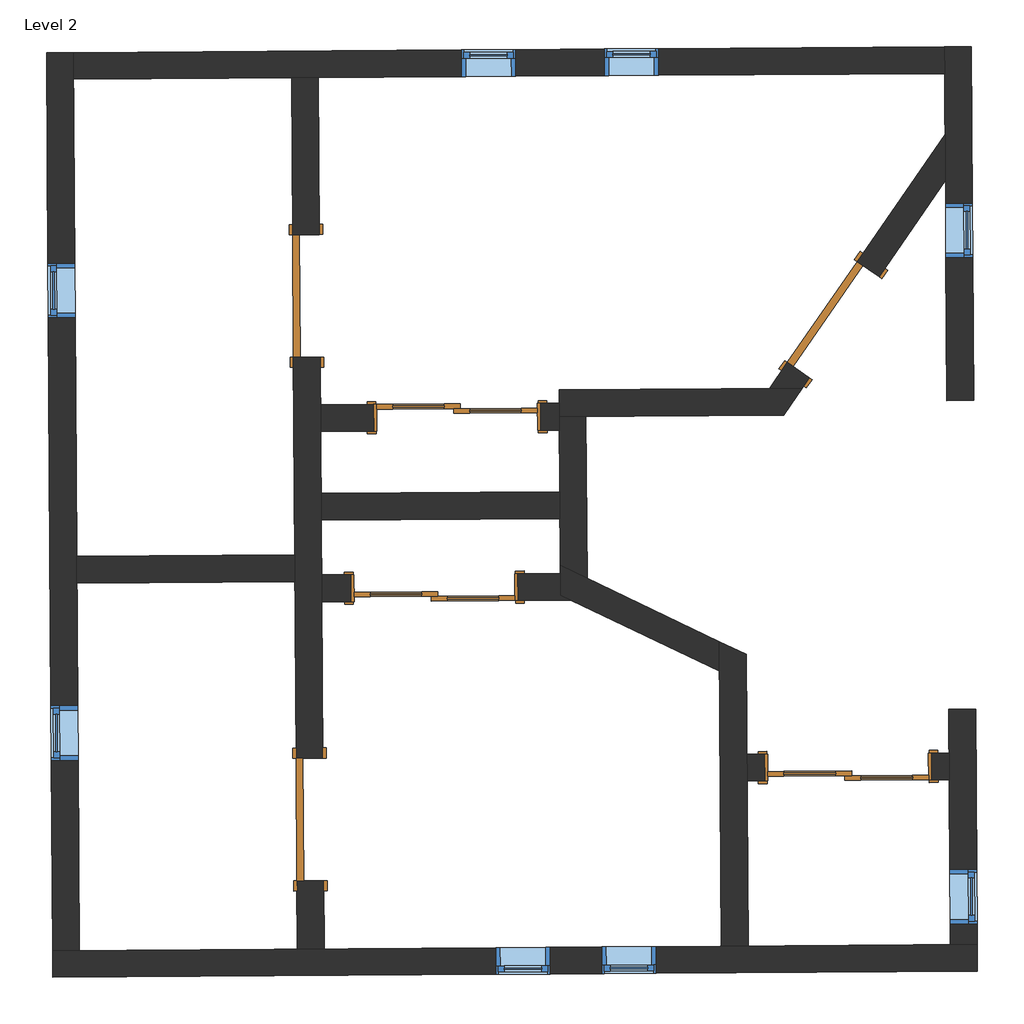
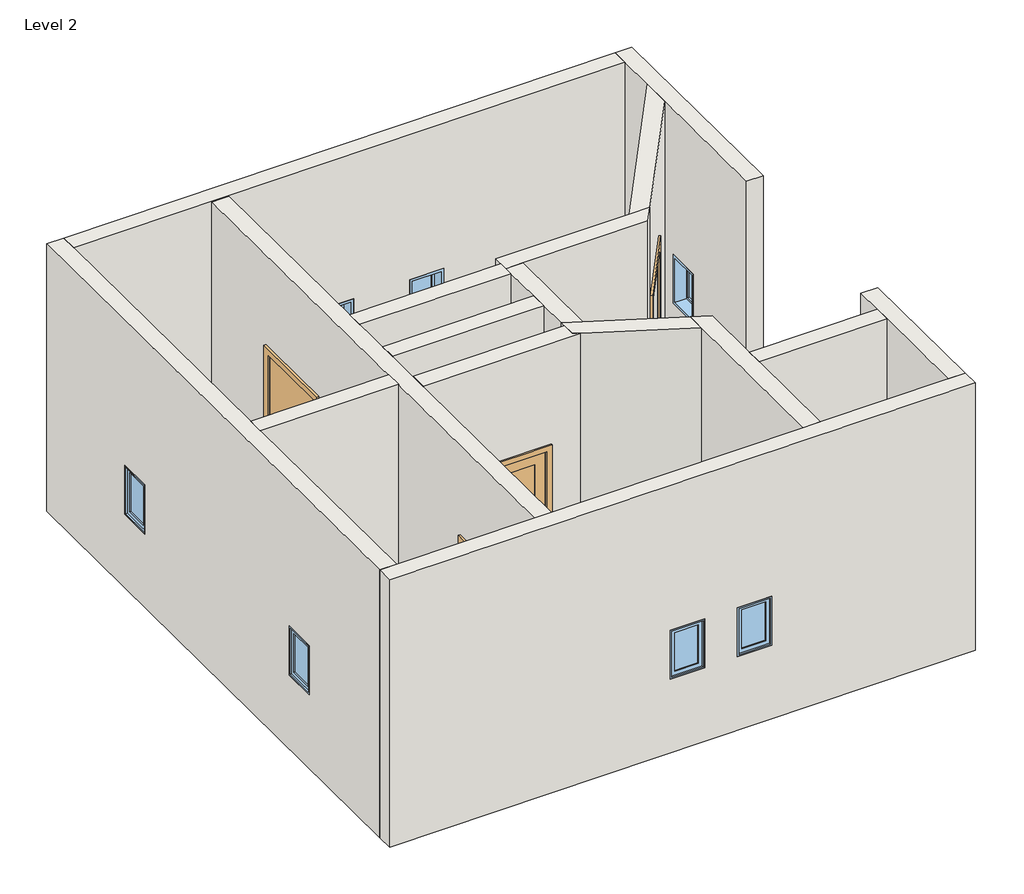
# One storey: 16 walls, 8 windows, 6 doors.
"""IFC4 building model written with IfcOpenShell, lengths in millimetres."""

import ifcopenshell
import ifcopenshell.guid

model = None  # the IFC model being written
_history = None  # IfcOwnerHistory: only IFC2X3 demands one
_inside = {}  # id of a spatial element -> (the spatial element, [elements in it])
_under = {}  # id of a project, library or spatial element -> (it, [spatial elements below it])
_declared = {}  # id of a project -> (the project, [libraries it declares])
_typed = {}  # id of a type object -> (the type object, [elements of that type])
_made_of = {}  # id of a material, layer set ... -> (it, [elements and type objects made of it])


def new_model(schema):
    """Start an empty IFC model of exactly this schema.

    Asked for "IFC4X3", IfcOpenShell would pick the latest addendum, in which some entities
    have other attributes; the version numbers below select the first issue.
    IFC2X3 requires an IfcOwnerHistory on every rooted entity: one is made here for all.
    """
    global model, _history
    if schema == "IFC4X3":
        model = ifcopenshell.file(schema_version=(4, 3, 0, 0))
    else:
        model = ifcopenshell.file(schema=schema)
    _inside.clear()
    _under.clear()
    _declared.clear()
    _typed.clear()
    _made_of.clear()
    _history = None
    if model.schema == "IFC2X3":
        org = make("IfcOrganization", Name="unknown")
        user = make(
            "IfcPersonAndOrganization",
            ThePerson=make("IfcPerson", FamilyName="unknown"),
            TheOrganization=org,
        )
        app = make(
            "IfcApplication",
            ApplicationDeveloper=org,
            Version="unknown",
            ApplicationFullName="unknown",
            ApplicationIdentifier="unknown",
        )
        _history = make(
            "IfcOwnerHistory",
            OwningUser=user,
            OwningApplication=app,
            ChangeAction="ADDED",
            CreationDate=0,
        )
    return model


def make(cls, **values):
    """One entity of the class cls with the attributes given. An attribute that is None is left unset."""
    return model.create_entity(
        cls, **{name: value for name, value in values.items() if value is not None}
    )


def rooted(cls, **values):
    """An entity with a GlobalId (a new one), such as an element, a storey or a relation."""
    return make(cls, GlobalId=ifcopenshell.guid.new(), OwnerHistory=_history, **values)


def si_unit(unit_type, name, prefix=None):
    """IfcSIUnit, for example si_unit("LENGTHUNIT", "METRE", prefix="MILLI")."""
    return make("IfcSIUnit", UnitType=unit_type, Prefix=prefix, Name=name)


def assignment(units):
    """IfcUnitAssignment: the units of a project."""
    return None if units is None else make("IfcUnitAssignment", Units=units)


def point(xyz):
    """IfcCartesianPoint."""
    return None if xyz is None else make("IfcCartesianPoint", Coordinates=xyz)


def direction(xyz):
    """IfcDirection."""
    return None if xyz is None else make("IfcDirection", DirectionRatios=xyz)


def frame(location, z_axis=None, x_axis=None):
    """IfcAxis2Placement3D, a coordinate frame: its origin and axes. An axis left out is left unset."""
    return make(
        "IfcAxis2Placement3D",
        Location=point(location),
        Axis=direction(z_axis),
        RefDirection=direction(x_axis),
    )


def origin():
    """The frame at (0, 0, 0) with its axes left unset."""
    return frame((0.0, 0.0, 0.0))


def origin_with_axes():
    """The frame at (0, 0, 0) with the z axis (0, 0, 1) and the x axis (1, 0, 0) written out."""
    return frame((0.0, 0.0, 0.0), z_axis=(0.0, 0.0, 1.0), x_axis=(1.0, 0.0, 0.0))


def place(relative_to, where):
    """IfcLocalPlacement: puts the frame where relative to a parent placement (None: the world)."""
    return make(
        "IfcLocalPlacement", PlacementRelTo=relative_to, RelativePlacement=where
    )


def context(
    kind, dimensions, precision=None, world=None, true_north=None, identifier=None
):
    """IfcGeometricRepresentationContext, for example the 3D "Model" context."""
    return make(
        "IfcGeometricRepresentationContext",
        ContextIdentifier=identifier,
        ContextType=kind,
        CoordinateSpaceDimension=dimensions,
        Precision=precision,
        WorldCoordinateSystem=world,
        TrueNorth=true_north,
    )


def project(units=None, contexts=None):
    """IfcProject with its units and contexts."""
    return rooted(
        "IfcProject",
        Name="project",
        RepresentationContexts=contexts,
        UnitsInContext=assignment(units),
    )


def spatial(cls, under=None, at=None, **own):
    """A site, building, storey or space (cls), placed at a placement, below another one or the project."""
    s = rooted(cls, ObjectPlacement=at, **own)
    if under is not None:
        _under.setdefault(under.id(), (under, []))[1].append(s)
    return s


def polyline(points):
    """IfcPolyline through the points."""
    return make("IfcPolyline", Points=[point(p) for p in points])


def outline(outer, holes=None, kind="AREA"):
    """IfcArbitraryClosedProfileDef: a profile drawn as a closed curve; with holes, ...WithVoids."""
    if holes is None:
        return make("IfcArbitraryClosedProfileDef", ProfileType=kind, OuterCurve=outer)
    return make(
        "IfcArbitraryProfileDefWithVoids",
        ProfileType=kind,
        OuterCurve=outer,
        InnerCurves=holes,
    )


def extrude(swept, where, along, depth):
    """IfcExtrudedAreaSolid: the profile swept, set in the frame where, extruded along a direction by depth."""
    return make(
        "IfcExtrudedAreaSolid",
        SweptArea=swept,
        Position=where,
        ExtrudedDirection=direction(along),
        Depth=depth,
    )


def faces_of(points, faces, orient=None, outer=None):
    """IfcFace entities. A face is a list of loops; a loop is a list of indices into points, from 0.

    orient and outer hold one flag for each loop. By default every Orientation is true, the
    first loop of a face is its IfcFaceOuterBound and the others are IfcFaceBound.
    """
    made = []
    for i, loops in enumerate(faces):
        bounds = []
        for j, loop in enumerate(loops):
            is_outer = j == 0 if outer is None else outer[i][j]
            bounds.append(
                make(
                    "IfcFaceOuterBound" if is_outer else "IfcFaceBound",
                    Bound=make("IfcPolyLoop", Polygon=[points[k] for k in loop]),
                    Orientation=True if orient is None else orient[i][j],
                )
            )
        made.append(make("IfcFace", Bounds=bounds))
    return made


def faceted_brep(points, faces, orient=None, outer=None, voids=None):
    """IfcFacetedBrep: a solid bounded by flat faces; with voids (closed shells), ...WithVoids."""
    shared = [point(p) for p in points]
    hull = make("IfcClosedShell", CfsFaces=faces_of(shared, faces, orient, outer))
    if voids is None:
        return make("IfcFacetedBrep", Outer=hull)
    return make(
        "IfcFacetedBrepWithVoids",
        Outer=hull,
        Voids=[
            make(cls, CfsFaces=faces_of(shared, fs, o, b)) for cls, fs, o, b in voids
        ],
    )


def shape(context_of_items, identifier, shape_type, items):
    """IfcShapeRepresentation: the items that make up one representation, for example the "Body"."""
    return make(
        "IfcShapeRepresentation",
        ContextOfItems=context_of_items,
        RepresentationIdentifier=identifier,
        RepresentationType=shape_type,
        Items=items,
    )


def source(mapping_origin, context_of_items, identifier, shape_type, items):
    """IfcRepresentationMap: a shape defined once, which mapped items show again and again."""
    return make(
        "IfcRepresentationMap",
        MappingOrigin=mapping_origin,
        MappedRepresentation=shape(context_of_items, identifier, shape_type, items),
    )


def transform(
    local_origin,
    x_axis=None,
    y_axis=None,
    z_axis=None,
    scale=None,
    scale2=None,
    scale3=None,
    uniform=True,
):
    """IfcCartesianTransformationOperator3D, or its non-uniform kind. x_axis, y_axis, z_axis: its Axis1, 2, 3."""
    if uniform:
        return make(
            "IfcCartesianTransformationOperator3D",
            Axis1=direction(x_axis),
            Axis2=direction(y_axis),
            LocalOrigin=point(local_origin),
            Scale=scale,
            Axis3=direction(z_axis),
        )
    return make(
        "IfcCartesianTransformationOperator3DnonUniform",
        Axis1=direction(x_axis),
        Axis2=direction(y_axis),
        LocalOrigin=point(local_origin),
        Scale=scale,
        Axis3=direction(z_axis),
        Scale2=scale2,
        Scale3=scale3,
    )


def mapped(mapping_source, mapping_target):
    """IfcMappedItem: shows the shape of a source again, moved by a transform."""
    return make(
        "IfcMappedItem", MappingSource=mapping_source, MappingTarget=mapping_target
    )


def made_of(thing, what):
    """Note that an element or type object is made of a material, layer set ...; save() writes the relation."""
    if what is not None:
        _made_of.setdefault(what.id(), (what, []))[1].append(thing)
    return thing


def element(
    cls,
    number,
    at=None,
    inside=None,
    cuts=None,
    type_object=None,
    material=None,
    context=None,
    identifier="Body",
    shape_type=None,
    held_by="IfcProductDefinitionShape",
    body=None,
    shapes=None,
    **own,
):
    """One element of the class cls, such as IfcWall. Its Tag is "e" and its number.

    at: its placement. inside: the storey or other place that contains it. cuts: it is an
    opening in that element (IfcRelVoidsElement). A single representation is given by context,
    identifier, shape_type and body (its items); several are given by shapes. held_by: the class
    of the entity that holds the representations. save() writes the other relations.
    """
    e = rooted(cls, Tag="e%d" % number, ObjectPlacement=at, **own)
    if body is not None:
        shapes = [shape(context, identifier, shape_type, body)]
    if shapes is not None:
        e.Representation = make(held_by, Representations=shapes)
    if inside is not None:
        _inside.setdefault(inside.id(), (inside, []))[1].append(e)
    if cuts is not None:
        rooted(
            "IfcRelVoidsElement", RelatingBuildingElement=cuts, RelatedOpeningElement=e
        )
    if type_object is not None:
        _typed.setdefault(type_object.id(), (type_object, []))[1].append(e)
    return made_of(e, material)


def aggregate(whole, parts):
    """IfcRelAggregates: a whole, such as a stair, and the parts it consists of."""
    return rooted("IfcRelAggregates", RelatingObject=whole, RelatedObjects=parts)


def save(model, path):
    """Write the relations noted so far, then the file.

    IfcRelAggregates (storeys below a building ...), IfcRelContainedInSpatialStructure (elements
    in a storey), IfcRelDefinesByType, IfcRelAssociatesMaterial and IfcRelDeclares: one each for
    every whole, place, type object, material and project.
    """
    for whole, parts in _under.values():
        aggregate(whole, parts)
    for where, things in _inside.values():
        rooted(
            "IfcRelContainedInSpatialStructure",
            RelatedElements=things,
            RelatingStructure=where,
        )
    for kind, things in _typed.values():
        rooted("IfcRelDefinesByType", RelatedObjects=things, RelatingType=kind)
    for what, things in _made_of.values():
        rooted("IfcRelAssociatesMaterial", RelatedObjects=things, RelatingMaterial=what)
    for by, libraries in _declared.values():
        rooted("IfcRelDeclares", RelatingContext=by, RelatedDefinitions=libraries)
    model.write(path)


def m_door_interior_double_sliding_2_panel_wood_1200_x_2000mm_2523b4d6(model_context):
    return source(origin(), model_context, "Body", "SweptSolid", [
        extrude(outline(polyline([(480.0, 38.4916667), (94.6, 38.4916667), (94.6, 50.1583333), (480.0, 50.1583333), (480.0, 38.4916667)])), frame((0.0, 0.0, 1014.4), z_axis=(0.0, 0.0, 1.0), x_axis=(1.0, 0.0, 0.0)), (0.0, 0.0, 1.0), 865.6),
        extrude(outline(polyline([(480.0, 38.4916667), (94.6, 38.4916667), (94.6, 50.1583333), (480.0, 50.1583333), (480.0, 38.4916667)])), frame((0.0, 0.0, 230.0), z_axis=(0.0, 0.0, 1.0), x_axis=(1.0, 0.0, 0.0)), (0.0, 0.0, 1.0), 584.4),
        extrude(outline(polyline([(2000.0, -25.4), (0.0, -25.4), (0.0, 600.0), (2000.0, 600.0), (2000.0, -25.4)]), holes=[polyline([(1880.0, 94.6), (1880.0, 480.0), (1014.4, 480.0), (1014.4, 94.6), (1880.0, 94.6)]), polyline([(814.4, 94.6), (814.4, 480.0), (230.0, 480.0), (230.0, 94.6), (814.4, 94.6)])]), frame((0.0, 26.825, 0.0), z_axis=(0.0, 1.0, 0.0), x_axis=(0.0, 0.0, 1.0)), (0.0, 0.0, 1.0), 35.0),
        extrude(outline(polyline([(-94.6, 73.4916667), (-480.0, 73.4916667), (-480.0, 85.1583333), (-94.6, 85.1583333), (-94.6, 73.4916667)])), frame((0.0, 0.0, 1014.4), z_axis=(0.0, 0.0, 1.0), x_axis=(1.0, 0.0, 0.0)), (0.0, 0.0, 1.0), 865.6),
        extrude(outline(polyline([(-94.6, 73.4916667), (-480.0, 73.4916667), (-480.0, 85.1583333), (-94.6, 85.1583333), (-94.6, 73.4916667)])), frame((0.0, 0.0, 230.0), z_axis=(0.0, 0.0, 1.0), x_axis=(1.0, 0.0, 0.0)), (0.0, 0.0, 1.0), 584.4),
        extrude(outline(polyline([(2000.0, -600.0), (0.0, -600.0), (0.0, 25.4), (2000.0, 25.4), (2000.0, -600.0)]), holes=[polyline([(1880.0, -480.0), (1880.0, -94.6), (1014.4, -94.6), (1014.4, -480.0), (1880.0, -480.0)]), polyline([(814.4, -480.0), (814.4, -94.6), (230.0, -94.6), (230.0, -480.0), (814.4, -480.0)])]), frame((0.0, 61.825, 0.0), z_axis=(0.0, 1.0, 0.0), x_axis=(0.0, 0.0, 1.0)), (0.0, 0.0, 1.0), 35.0),
        extrude(outline(polyline([(0.0, 600.0), (0.0, 625.0), (2025.0, 625.0), (2025.0, -625.0), (0.0, -625.0), (0.0, -600.0), (2000.0, -600.0), (2000.0, 600.0), (0.0, 600.0)])), frame((0.0, -103.175, 0.0), z_axis=(0.0, 1.0, 0.0), x_axis=(0.0, 0.0, 1.0)), (0.0, 0.0, 1.0), 200.0),
        extrude(outline(polyline([(0.0, 606.35), (0.0, 671.35), (2071.35, 671.35), (2071.35, -671.35), (0.0, -671.35), (0.0, -606.35), (2006.35, -606.35), (2006.35, 606.35), (0.0, 606.35)])), frame((0.0, -123.175, 0.0), z_axis=(0.0, 1.0, 0.0), x_axis=(0.0, 0.0, 1.0)), (0.0, 0.0, 1.0), 20.0),
        extrude(outline(polyline([(0.0, 606.35), (0.0, 671.35), (2071.35, 671.35), (2071.35, -671.35), (0.0, -671.35), (0.0, -606.35), (2006.35, -606.35), (2006.35, 606.35), (0.0, 606.35)])), frame((0.0, 96.825, 0.0), z_axis=(0.0, 1.0, 0.0), x_axis=(0.0, 0.0, 1.0)), (0.0, 0.0, 1.0), 20.0),
    ])


def m_single_flush_0915_x_2134mm_6a9e8738(model_context):
    return source(origin(), model_context, "Body", "SweptSolid", [
        extrude(outline(polyline([(2210.0, -533.5), (0.0, -533.5), (0.0, -457.5), (2134.0, -457.5), (2134.0, 457.5), (0.0, 457.5), (0.0, 533.5), (2210.0, 533.5), (2210.0, -533.5)])), frame((0.0, 100.0, 0.0), z_axis=(0.0, 1.0, 0.0), x_axis=(0.0, 0.0, 1.0)), (0.0, 0.0, 1.0), 25.0),
        extrude(outline(polyline([(2210.0, 533.5), (2210.0, -533.5), (0.0, -533.5), (0.0, -457.5), (2134.0, -457.5), (2134.0, 457.5), (0.0, 457.5), (0.0, 533.5), (2210.0, 533.5)])), frame((0.0, -125.0, 0.0), z_axis=(0.0, 1.0, 0.0), x_axis=(0.0, 0.0, 1.0)), (0.0, 0.0, 1.0), 25.0),
        extrude(outline(polyline([(457.5, 49.0), (-457.5, 49.0), (-457.5, 100.0), (457.5, 100.0), (457.5, 49.0)])), origin_with_axes(), (0.0, 0.0, 1.0), 2134.0),
    ])


def m_single_flush_0915_x_2134mm_727434cd(model_context):
    return source(origin(), model_context, "Body", "SweptSolid", [
        extrude(outline(polyline([(2210.0, -533.5), (0.0, -533.5), (0.0, -457.5), (2134.0, -457.5), (2134.0, 457.5), (0.0, 457.5), (0.0, 533.5), (2210.0, 533.5), (2210.0, -533.5)])), frame((0.0, -125.0, 0.0), z_axis=(0.0, 1.0, 0.0), x_axis=(0.0, 0.0, 1.0)), (0.0, 0.0, 1.0), 25.0),
        extrude(outline(polyline([(2210.0, 533.5), (2210.0, -533.5), (0.0, -533.5), (0.0, -457.5), (2134.0, -457.5), (2134.0, 457.5), (0.0, 457.5), (0.0, 533.5), (2210.0, 533.5)])), frame((0.0, 100.0, 0.0), z_axis=(0.0, 1.0, 0.0), x_axis=(0.0, 0.0, 1.0)), (0.0, 0.0, 1.0), 25.0),
        extrude(outline(polyline([(457.5, -49.0), (457.5, -100.0), (-457.5, -100.0), (-457.5, -49.0), (457.5, -49.0)])), origin_with_axes(), (0.0, 0.0, 1.0), 2134.0),
    ])


def m_fixed_0406_x_0610mm_8205b201(model_context):
    return source(origin(), model_context, "Body", "SweptSolid", [
        extrude(outline(polyline([(-140.0, 78.0), (140.0, 78.0), (140.0, 66.0), (-140.0, 66.0), (-140.0, 78.0)])), frame((0.0, 0.0, 978.0), z_axis=(0.0, 0.0, 1.0), x_axis=(1.0, 0.0, 0.0)), (0.0, 0.0, 1.0), 484.0),
        extrude(outline(polyline([(1506.0, -184.0), (934.0, -184.0), (934.0, 184.0), (1506.0, 184.0), (1506.0, -184.0)]), holes=[polyline([(1462.0, -140.0), (1462.0, 140.0), (978.0, 140.0), (978.0, -140.0), (1462.0, -140.0)])]), frame((0.0, 50.0, 0.0), z_axis=(0.0, 1.0, 0.0), x_axis=(0.0, 0.0, 1.0)), (0.0, 0.0, 1.0), 44.0),
        extrude(outline(polyline([(1525.0, -203.0), (915.0, -203.0), (915.0, 203.0), (1525.0, 203.0), (1525.0, -203.0)]), holes=[polyline([(1506.0, -184.0), (1506.0, 184.0), (934.0, 184.0), (934.0, -184.0), (1506.0, -184.0)])]), frame((0.0, 50.0, 0.0), z_axis=(0.0, 1.0, 0.0), x_axis=(0.0, 0.0, 1.0)), (0.0, 0.0, 1.0), 63.0),
        extrude(outline(polyline([(1525.0, -203.0), (915.0, -203.0), (915.0, 203.0), (1525.0, 203.0), (1525.0, -203.0)]), holes=[polyline([(1493.0, -171.0), (1493.0, 171.0), (947.0, 171.0), (947.0, -171.0), (1493.0, -171.0)])]), frame((0.0, -87.0, 0.0), z_axis=(0.0, 1.0, 0.0), x_axis=(0.0, 0.0, 1.0)), (0.0, 0.0, 1.0), 137.0),
    ])


model = new_model("IFC4")

# Units and contexts
model_context = context("Model", 3, world=origin())
ifc_project = project(units=[si_unit("LENGTHUNIT", "METRE", prefix="MILLI")], contexts=[model_context])

# Site, building, storey
site = spatial("IfcSite", under=ifc_project)
building = spatial("IfcBuilding", under=site)
storey = spatial("IfcBuildingStorey", under=building, Name="Level 2", Elevation=3048.0)

# Doors
placement = place(None, origin())
m_door_interior_double_sliding_2_panel_wood_1200_x_2000mm_shape = m_door_interior_double_sliding_2_panel_wood_1200_x_2000mm_2523b4d6(model_context)
element("IfcDoor", 1, ObjectType="M_Door-Interior-Double-Sliding-2_Panel-Wood : 1200 x 2000mm", at=placement, inside=storey, context=model_context, shape_type="MappedRepresentation", body=[
    mapped(m_door_interior_double_sliding_2_panel_wood_1200_x_2000mm_shape, transform((-71680.7342744, -7306.8218345, 3048.0), x_axis=(0.9999777944135733, 0.006664133834601911, 0.0), y_axis=(-0.006664133834601911, 0.9999777944135733, 0.0), z_axis=(0.0, 0.0, 1.0))),
])
element("IfcDoor", 2, ObjectType="M_Door-Interior-Double-Sliding-2_Panel-Wood : 1200 x 2000mm", at=placement, inside=storey, context=model_context, shape_type="MappedRepresentation", body=[
    mapped(m_door_interior_double_sliding_2_panel_wood_1200_x_2000mm_shape, transform((-71850.8195491, -8585.0827996, 3048.0), x_axis=(-0.9999777944135733, -0.006664133834601911, 0.0), y_axis=(0.006664133834601911, -0.9999777944135733, 0.0), z_axis=(0.0, 0.0, 1.0))),
])
element("IfcDoor", 3, ObjectType="M_Door-Interior-Double-Sliding-2_Panel-Wood : 1200 x 2000mm", at=placement, inside=storey, context=model_context, shape_type="MappedRepresentation", body=[
    mapped(m_door_interior_double_sliding_2_panel_wood_1200_x_2000mm_shape, transform((-68760.728221, -9924.4626813, 3048.0), x_axis=(-0.9999777944135733, -0.006664133834601911, 0.0), y_axis=(0.006664133834601911, -0.9999777944135733, 0.0), z_axis=(0.0, 0.0, 1.0))),
])
m_single_flush_0915_x_2134mm_shape = m_single_flush_0915_x_2134mm_6a9e8738(model_context)
element("IfcDoor", 4, ObjectType="M_Single-Flush : 0915 x 2134mm", at=placement, inside=storey, context=model_context, shape_type="MappedRepresentation", body=[
    mapped(m_single_flush_0915_x_2134mm_shape, transform((-68872.1991372, -6581.0027274, 3048.0), x_axis=(0.5681047608958888, 0.8229562446736918, 0.0), y_axis=(-0.8229562446736918, 0.5681047608958888, 0.0), z_axis=(0.0, 0.0, 1.0))),
])
element("IfcDoor", 5, ObjectType="M_Single-Flush : 0915 x 2134mm", at=placement, inside=storey, context=model_context, shape_type="MappedRepresentation", body=[
    mapped(m_single_flush_0915_x_2134mm_shape, transform((-72805.9812977, -6403.1730367, 3048.0), x_axis=(-0.0066641338345986775, 0.9999777944135734, 0.0), y_axis=(-0.9999777944135734, -0.0066641338345986775, 0.0), z_axis=(0.0, 0.0, 1.0))),
])
m_single_flush_0915_x_2134mm_2_shape = m_single_flush_0915_x_2134mm_727434cd(model_context)
element("IfcDoor", 6, ObjectType="M_Single-Flush : 0915 x 2134mm", at=placement, inside=storey, context=model_context, shape_type="MappedRepresentation", body=[
    mapped(m_single_flush_0915_x_2134mm_2_shape, transform((-72779.9238848, -10313.1836822, 3048.0), x_axis=(0.0066641338345986775, -0.9999777944135734, 0.0), y_axis=(0.9999777944135734, 0.0066641338345986775, 0.0), z_axis=(0.0, 0.0, 1.0))),
])

# Walls
element("IfcWall", 7, ObjectType="Generic - 200mm", at=placement, inside=storey, context=model_context, shape_type="Brep", body=[
    faceted_brep([(-67796.791513, -11246.7961526, 3048.0), (-67996.7870719, -11248.1289794, 3048.0), (-69506.9597289, -11258.1931955, 3048.0), (-69706.9552878, -11259.5260223, 3048.0), (-72673.4832208, -11279.2958005, 3048.0), (-72873.4787797, -11280.6286272, 3048.0), (-74502.2426112, -11291.4831684, 3048.0), (-74702.2381701, -11292.8159952, 3048.0), (-74702.2381701, -11292.8159952, 6372.225), (-74502.2426112, -11291.4831684, 6372.225), (-69706.9552878, -11259.5260223, 6372.225), (-69506.9597289, -11258.1931955, 6372.225), (-67996.7870719, -11248.1289794, 6372.225), (-67796.791513, -11246.7961526, 6372.225), (-70987.223762, -11268.0580922, 3963.0), (-70987.223762, -11268.0580922, 4573.0), (-71393.2147465, -11270.7637306, 4573.0), (-71393.2147465, -11270.7637306, 3963.0), (-70195.592889, -11262.782441, 3963.0), (-70195.592889, -11262.782441, 4573.0), (-70601.5838736, -11265.4880793, 4573.0), (-70601.5838736, -11265.4880793, 3963.0), (-67795.4586862, -11446.7917115, 3048.0), (-67795.4586862, -11446.7917115, 6372.225), (-74700.9053433, -11492.8115541, 6372.225), (-74700.9053433, -11492.8115541, 3048.0), (-70985.8909352, -11468.0536511, 3963.0), (-71391.8819198, -11470.7592894, 3963.0), (-71391.8819198, -11470.7592894, 4573.0), (-70985.8909352, -11468.0536511, 4573.0), (-70194.2600623, -11462.7779999, 3963.0), (-70600.2510468, -11465.4836382, 3963.0), (-70600.2510468, -11465.4836382, 4573.0), (-70194.2600623, -11462.7779999, 4573.0)], [[[0, 1, 2, 3, 4, 5, 6, 7, 8, 9, 10, 11, 12, 13], [14, 15, 16, 17], [18, 19, 20, 21]], [[22, 23, 24, 25], [26, 27, 28, 29], [30, 31, 32, 33]], [[8, 7, 25, 24]], [[0, 13, 23, 22]], [[15, 14, 26, 29]], [[16, 15, 29, 28]], [[17, 16, 28, 27]], [[14, 17, 27, 26]], [[19, 18, 30, 33]], [[20, 19, 33, 32]], [[21, 20, 32, 31]], [[18, 21, 31, 30]], [[7, 6, 5, 4, 3, 2, 1, 0, 22, 25]], [[13, 12, 11, 10, 9, 8, 24, 23]]]),
])
element("IfcWall", 8, ObjectType="Generic - 200mm", at=placement, inside=storey, context=model_context, shape_type="Brep", body=[
    faceted_brep([(-74502.2426112, -11291.4831684, 3048.0), (-74520.5249623, -8548.1491441, 3048.0), (-74521.857789, -8348.1535853, 3048.0), (-74545.5968003, -4786.0276291, 3048.0), (-74546.9296271, -4586.0320702, 3048.0), (-74546.9296271, -4586.0320702, 6372.225), (-74545.5968003, -4786.0276291, 6372.225), (-74521.857789, -8348.1535853, 6372.225), (-74520.5249623, -8548.1491441, 6372.225), (-74502.2426112, -11291.4831684, 6372.225), (-74533.7386405, -6565.3881165, 3963.0), (-74533.7386405, -6565.3881165, 4573.0), (-74536.4442789, -6159.3971319, 4573.0), (-74536.4442789, -6159.3971319, 3963.0), (-74511.7136445, -9870.3197839, 3963.0), (-74511.7136445, -9870.3197839, 4573.0), (-74514.4192829, -9464.3287994, 4573.0), (-74514.4192829, -9464.3287994, 3963.0), (-74702.2381701, -11292.8159952, 3048.0), (-74702.2381701, -11292.8159952, 6372.225), (-74746.9251859, -4587.364897, 6372.225), (-74746.9251859, -4587.364897, 3048.0), (-74733.7341994, -6566.7209432, 3963.0), (-74736.4398378, -6160.7299587, 3963.0), (-74736.4398378, -6160.7299587, 4573.0), (-74733.7341994, -6566.7209432, 4573.0), (-74711.7092034, -9871.6526107, 3963.0), (-74714.4148417, -9465.6616262, 3963.0), (-74714.4148417, -9465.6616262, 4573.0), (-74711.7092034, -9871.6526107, 4573.0)], [[[0, 1, 2, 3, 4, 5, 6, 7, 8, 9], [10, 11, 12, 13], [14, 15, 16, 17]], [[18, 19, 20, 21], [22, 23, 24, 25], [26, 27, 28, 29]], [[4, 3, 2, 1, 0, 18, 21]], [[9, 8, 7, 6, 5, 20, 19]], [[0, 9, 19, 18]], [[5, 4, 21, 20]], [[11, 10, 22, 25]], [[12, 11, 25, 24]], [[13, 12, 24, 23]], [[10, 13, 23, 22]], [[15, 14, 26, 29]], [[16, 15, 29, 28]], [[17, 16, 28, 27]], [[14, 17, 27, 26]]]),
])
element("IfcWall", 9, ObjectType="Generic - 200mm", at=placement, inside=storey, context=model_context, shape_type="Brep", body=[
    faceted_brep([(-74545.5968003, -4786.0276291, 3048.0), (-72916.8329687, -4775.1730879, 3048.0), (-72716.8374099, -4773.8402611, 3048.0), (-68040.141261, -4742.67344, 3048.0), (-68040.141261, -4742.67344, 6372.225), (-74545.5968003, -4786.0276291, 6372.225), (-70581.4848277, -4759.6096698, 3963.0), (-70581.4848277, -4759.6096698, 4573.0), (-70175.4938431, -4756.9040314, 4573.0), (-70175.4938431, -4756.9040314, 3963.0), (-71648.2611388, -4766.7189677, 3963.0), (-71648.2611388, -4766.7189677, 4573.0), (-71242.2701542, -4764.0133294, 4573.0), (-71242.2701542, -4764.0133294, 3963.0), (-74546.9296271, -4586.0320702, 3048.0), (-74546.9296271, -4586.0320702, 6372.225), (-68041.4740877, -4542.6778811, 6372.225), (-68041.4740877, -4542.6778811, 3048.0), (-70582.8176544, -4559.6141109, 3963.0), (-70176.8266699, -4556.9084725, 3963.0), (-70176.8266699, -4556.9084725, 4573.0), (-70582.8176544, -4559.6141109, 4573.0), (-71649.5939655, -4566.7234088, 3963.0), (-71243.602981, -4564.0177705, 3963.0), (-71243.602981, -4564.0177705, 4573.0), (-71649.5939655, -4566.7234088, 4573.0)], [[[0, 1, 2, 3, 4, 5], [6, 7, 8, 9], [10, 11, 12, 13]], [[14, 15, 16, 17], [18, 19, 20, 21], [22, 23, 24, 25]], [[3, 2, 1, 0, 14, 17]], [[5, 4, 16, 15]], [[0, 5, 15, 14]], [[7, 6, 18, 21]], [[8, 7, 21, 20]], [[9, 8, 20, 19]], [[6, 9, 19, 18]], [[11, 10, 22, 25]], [[12, 11, 25, 24]], [[13, 12, 24, 23]], [[10, 13, 23, 22]], [[4, 3, 17, 16]]]),
])
element("IfcWall", 10, ObjectType="Generic - 200mm", at=placement, inside=storey, context=model_context, shape_type="Brep", body=[
    faceted_brep([(-68041.4740877, -4542.6778811, 3048.0), (-68040.141261, -4742.67344, 3048.0), (-68037.1248916, -5195.2907613, 3048.0), (-68034.801179, -5543.9723775, 3048.0), (-68023.8607483, -7185.6242487, 3048.0), (-68023.8607483, -7185.6242487, 6372.225), (-68034.801179, -5543.9723775, 6372.225), (-68037.1248916, -5195.2907613, 6372.225), (-68040.141261, -4742.67344, 6372.225), (-68041.4740877, -4542.6778811, 6372.225), (-68033.6870305, -5711.1544624, 3963.0), (-68033.6870305, -5711.1544624, 4573.0), (-68030.9813921, -6117.1454469, 4573.0), (-68030.9813921, -6117.1454469, 3963.0), (-67841.4785288, -4541.3450544, 3048.0), (-67841.4785288, -4541.3450544, 6372.225), (-67823.8651894, -7184.2914219, 6372.225), (-67823.8651894, -7184.2914219, 3048.0), (-67833.6914716, -5709.8216356, 3963.0), (-67830.9858333, -6115.8126201, 3963.0), (-67830.9858333, -6115.8126201, 4573.0), (-67833.6914716, -5709.8216356, 4573.0)], [[[0, 1, 2, 3, 4, 5, 6, 7, 8, 9], [10, 11, 12, 13]], [[14, 15, 16, 17], [18, 19, 20, 21]], [[4, 3, 2, 1, 0, 14, 17]], [[5, 4, 17, 16]], [[9, 8, 7, 6, 5, 16, 15]], [[11, 10, 18, 21]], [[12, 11, 21, 20]], [[13, 12, 20, 19]], [[10, 13, 19, 18]], [[0, 9, 15, 14]]]),
])
element("IfcWall", 11, ObjectType="Generic - 200mm", at=placement, inside=storey, context=model_context, shape_type="Brep", body=[
    faceted_brep([(-67796.791513, -11246.7961526, 3048.0), (-67808.4990553, -9490.0363627, 3048.0), (-67808.4990553, -9490.0363627, 6372.225), (-67796.791513, -11246.7961526, 6372.225), (-67800.5247608, -10686.6085922, 3963.0), (-67797.8191224, -11092.5995767, 3963.0), (-67797.8191224, -11092.5995767, 4573.0), (-67800.5247608, -10686.6085922, 4573.0), (-67996.7870719, -11248.1289794, 3048.0), (-67996.7870719, -11248.1289794, 6372.225), (-68004.9966377, -10016.2534232, 6372.225), (-68006.3294645, -9816.2578643, 6372.225), (-68008.4946142, -9491.3691895, 6372.225), (-68008.4946142, -9491.3691895, 3048.0), (-68006.3294645, -9816.2578643, 3048.0), (-68004.9966377, -10016.2534232, 3048.0), (-68000.5203197, -10687.9414189, 3963.0), (-68000.5203197, -10687.9414189, 4573.0), (-67997.8146813, -11093.9324035, 4573.0), (-67997.8146813, -11093.9324035, 3963.0)], [[[0, 1, 2, 3], [4, 5, 6, 7]], [[8, 9, 10, 11, 12, 13, 14, 15], [16, 17, 18, 19]], [[1, 0, 8, 15, 14, 13]], [[2, 1, 13, 12]], [[3, 2, 12, 11, 10, 9]], [[0, 3, 9, 8]], [[17, 16, 4, 7]], [[18, 17, 7, 6]], [[19, 18, 6, 5]], [[16, 19, 5, 4]]]),
])
element("IfcWall", 12, ObjectType="Generic - 200mm", at=placement, inside=storey, context=model_context, shape_type="Brep", body=[
    faceted_brep([(-72876.872823, -10771.3399365, 5182.0), (-72876.872823, -10771.3399365, 3048.0), (-72873.4787797, -11280.6286272, 3048.0), (-72873.4787797, -11280.6286272, 6363.9898437), (-72916.8329687, -4775.1730879, 6363.9898437), (-72916.8329687, -4775.1730879, 3048.0), (-72909.0279183, -5946.3496092, 3048.0), (-72909.0279183, -5946.3496092, 5182.0), (-72902.9302359, -6861.3292911, 5182.0), (-72902.9302359, -6861.3292911, 3048.0), (-72893.0939575, -8337.2990441, 3048.0), (-72891.7611307, -8537.294603, 3048.0), (-72882.9705055, -9856.3602547, 3048.0), (-72882.9705055, -9856.3602547, 5182.0), (-72673.4832208, -11279.2958005, 3048.0), (-72676.8772642, -10770.0071098, 3048.0), (-72676.8772642, -10770.0071098, 5182.0), (-72682.9749466, -9855.0274279, 5182.0), (-72682.9749466, -9855.0274279, 3048.0), (-72690.7556283, -8687.5075204, 3048.0), (-72692.0884551, -8487.5119615, 3048.0), (-72694.8124138, -8078.7719286, 3048.0), (-72696.1452406, -7878.7763697, 3048.0), (-72699.2240704, -7416.7866287, 3048.0), (-72700.5568972, -7216.7910698, 3048.0), (-72702.934677, -6859.9964643, 3048.0), (-72702.934677, -6859.9964643, 5182.0), (-72709.0323595, -5945.0167824, 5182.0), (-72709.0323595, -5945.0167824, 3048.0), (-72716.8374099, -4773.8402611, 3048.0), (-72716.8374099, -4773.8402611, 6363.9898437), (-72673.4832208, -11279.2958005, 6363.9898437)], [[[0, 1, 2, 3, 4, 5, 6, 7, 8, 9, 10, 11, 12, 13]], [[14, 15, 16, 17, 18, 19, 20, 21, 22, 23, 24, 25, 26, 27, 28, 29, 30, 31]], [[3, 2, 14, 31]], [[5, 4, 30, 29]], [[7, 6, 28, 27]], [[8, 7, 27, 26]], [[9, 8, 26, 25]], [[16, 15, 1, 0]], [[17, 16, 0, 13]], [[18, 17, 13, 12]], [[29, 28, 6, 5]], [[2, 1, 15, 14]], [[12, 11, 10, 9, 25, 24, 23, 22, 21, 20, 19, 18]], [[4, 3, 31, 30]]]),
])
element("IfcWall", 13, ObjectType="Generic - 200mm", at=placement, inside=storey, context=model_context, shape_type="Brep", body=[
    faceted_brep([(-70918.7300364, -7304.9186941, 3048.0), (-70718.7344775, -7303.5858673, 3048.0), (-69242.7105492, -7293.7492279, 3048.0), (-69242.7105492, -7293.7492279, 6372.225), (-70718.7344775, -7303.5858673, 6372.225), (-70918.7300364, -7304.9186941, 6372.225), (-70920.0628632, -7104.9231352, 3048.0), (-70920.0628632, -7104.9231352, 6372.225), (-69348.1544742, -7094.4474947, 6372.225), (-69104.004978, -7092.8204136, 6372.225), (-69104.004978, -7092.8204136, 3048.0), (-69348.1544742, -7094.4474947, 3048.0), (-70919.3964498, -7204.9209146, 3048.0), (-70919.3964498, -7204.9209146, 6372.225)], [[[0, 1, 2, 3, 4, 5]], [[6, 7, 8, 9, 10, 11]], [[2, 1, 0, 12, 6, 11, 10]], [[5, 4, 3, 9, 8, 7, 13]], [[3, 2, 10, 9]], [[0, 5, 13, 7, 6, 12]]]),
])
element("IfcWall", 14, ObjectType="Generic - 200mm", at=placement, inside=storey, context=model_context, shape_type="Brep", body=[
    faceted_brep([(-68529.9955846, -6261.3107215, 5182.0), (-68529.9955846, -6261.3107215, 3048.0), (-68034.801179, -5543.9723775, 3048.0), (-68034.801179, -5543.9723775, 6372.225), (-69104.004978, -7092.8204136, 6372.225), (-69104.004978, -7092.8204136, 3048.0), (-69049.8114408, -7014.3156854, 3048.0), (-69049.8114408, -7014.3156854, 5182.0), (-68037.1248916, -5195.2907613, 3048.0), (-68694.5868335, -6147.6897693, 3048.0), (-68694.5868335, -6147.6897693, 5182.0), (-69214.4026897, -6900.6947332, 5182.0), (-69214.4026897, -6900.6947332, 3048.0), (-69348.1544742, -7094.4474947, 3048.0), (-69348.1544742, -7094.4474947, 6372.225), (-68037.1248916, -5195.2907613, 6372.225)], [[[0, 1, 2, 3, 4, 5, 6, 7]], [[8, 9, 10, 11, 12, 13, 14, 15]], [[6, 5, 13, 12]], [[2, 1, 9, 8]], [[4, 3, 15, 14]], [[5, 4, 14, 13]], [[3, 2, 8, 15]], [[10, 9, 1, 0]], [[11, 10, 0, 7]], [[12, 11, 7, 6]]]),
])
element("IfcWall", 15, ObjectType="Generic - 200mm", at=placement, inside=storey, context=model_context, shape_type="Brep", body=[
    faceted_brep([(-69722.1165345, -8984.5251792, 3048.0), (-69720.6343726, -9206.9290273, 3048.0), (-69706.9552878, -11259.5260223, 3048.0), (-69706.9552878, -11259.5260223, 6372.225), (-69720.6343726, -9206.9290273, 6372.225), (-69722.1165345, -8984.5251792, 6372.225), (-69521.4726109, -9080.4818591, 3048.0), (-69521.4726109, -9080.4818591, 6372.225), (-69516.5021215, -9826.3220805, 6372.225), (-69515.1692948, -10026.3176394, 6372.225), (-69506.9597289, -11258.1931955, 6372.225), (-69506.9597289, -11258.1931955, 3048.0), (-69515.1692948, -10026.3176394, 3048.0), (-69516.5021215, -9826.3220805, 3048.0)], [[[0, 1, 2, 3, 4, 5]], [[6, 7, 8, 9, 10, 11, 12, 13]], [[2, 1, 0, 6, 13, 12, 11]], [[5, 4, 3, 10, 9, 8, 7]], [[3, 2, 11, 10]], [[0, 5, 7, 6]]]),
])
element("IfcWall", 16, ObjectType="Generic - 200mm", at=placement, inside=storey, context=model_context, shape_type="Brep", body=[
    faceted_brep([(-70909.8446957, -8638.1967565, 3048.0), (-70832.629476, -8675.1244441, 3048.0), (-69720.6343726, -9206.9290273, 3048.0), (-69720.6343726, -9206.9290273, 6372.225), (-70832.629476, -8675.1244441, 6372.225), (-70909.8446957, -8638.1967565, 6372.225), (-70911.3268576, -8415.7929084, 3048.0), (-70911.3268576, -8415.7929084, 6372.225), (-70710.682934, -8511.7495883, 6372.225), (-69722.1165345, -8984.5251792, 6372.225), (-69722.1165345, -8984.5251792, 3048.0), (-70710.682934, -8511.7495883, 3048.0), (-70910.9280077, -8475.6418063, 3048.0), (-70910.9280077, -8475.6418063, 6372.225)], [[[0, 1, 2, 3, 4, 5]], [[6, 7, 8, 9, 10, 11]], [[2, 1, 0, 12, 6, 11, 10]], [[5, 4, 3, 9, 8, 7, 13]], [[3, 2, 10, 9]], [[0, 5, 13, 7, 6, 12]]]),
])
element("IfcWall", 17, ObjectType="Generic - 200mm", at=placement, inside=storey, context=model_context, shape_type="Brep", body=[
    faceted_brep([(-70918.7300364, -7304.9186941, 3048.0), (-70918.063623, -7404.9164735, 3048.0), (-70914.9847932, -7866.9062145, 3048.0), (-70913.6519664, -8066.9017734, 3048.0), (-70911.3268576, -8415.7929084, 3048.0), (-70911.3268576, -8415.7929084, 6372.225), (-70913.6519664, -8066.9017734, 6372.225), (-70914.9847932, -7866.9062145, 6372.225), (-70918.063623, -7404.9164735, 6372.225), (-70918.7300364, -7304.9186941, 6372.225), (-70718.7344775, -7303.5858673, 3048.0), (-70718.7344775, -7303.5858673, 6372.225), (-70710.682934, -8511.7495883, 6372.225), (-70710.682934, -8511.7495883, 3048.0)], [[[0, 1, 2, 3, 4, 5, 6, 7, 8, 9]], [[10, 11, 12, 13]], [[4, 3, 2, 1, 0, 10, 13]], [[9, 8, 7, 6, 5, 12, 11]], [[0, 9, 11, 10]], [[5, 4, 13, 12]]]),
])
element("IfcWall", 18, ObjectType="Generic - 200mm", at=placement, inside=storey, context=model_context, shape_type="SweptSolid", body=[
    extrude(outline(polyline([(-74521.857789, -8348.1535853), (-72893.0939575, -8337.2990441), (-72891.7611307, -8537.294603), (-74520.5249623, -8548.1491441), (-74521.857789, -8348.1535853)])), frame((0.0, 0.0, 3048.0), z_axis=(0.0, 0.0, 1.0), x_axis=(1.0, 0.0, 0.0)), (0.0, 0.0, 1.0), 3324.225),
])
element("IfcWall", 19, ObjectType="Generic - 200mm", at=placement, inside=storey, context=model_context, shape_type="Brep", body=[
    faceted_brep([(-72700.5568972, -7216.7910698, 6372.225), (-70919.3964498, -7204.9209146, 6372.225), (-70919.3964498, -7204.9209146, 3048.0), (-71056.3934076, -7205.833901, 3048.0), (-71056.3934076, -7205.833901, 5073.0), (-72306.3656506, -7214.1640682, 5073.0), (-72306.3656506, -7214.1640682, 3048.0), (-72700.5568972, -7216.7910698, 3048.0), (-70918.063623, -7404.9164735, 6372.225), (-72699.2240704, -7416.7866287, 6372.225), (-72699.2240704, -7416.7866287, 3048.0), (-72305.0328239, -7414.1596271, 3048.0), (-72305.0328239, -7414.1596271, 5073.0), (-71055.0605809, -7405.8294598, 5073.0), (-71055.0605809, -7405.8294598, 3048.0), (-70918.063623, -7404.9164735, 3048.0), (-70918.7300364, -7304.9186941, 3048.0), (-70918.7300364, -7304.9186941, 6372.225)], [[[0, 1, 2, 3, 4, 5, 6, 7]], [[8, 9, 10, 11, 12, 13, 14, 15]], [[2, 16, 15, 14, 3]], [[10, 7, 6, 11]], [[1, 0, 9, 8, 17]], [[0, 7, 10, 9]], [[2, 1, 17, 8, 15, 16]], [[13, 4, 3, 14]], [[4, 13, 12, 5]], [[5, 12, 11, 6]]]),
])
element("IfcWall", 20, ObjectType="Generic - 200mm", at=placement, inside=storey, context=model_context, shape_type="Brep", body=[
    faceted_brep([(-72692.0884551, -8487.5119615, 6372.225), (-70910.9280077, -8475.6418063, 6372.225), (-70910.9280077, -8475.6418063, 3048.0), (-71226.5209996, -8477.745007, 3048.0), (-71226.5209996, -8477.745007, 5073.0), (-72476.4932426, -8486.0751743, 5073.0), (-72476.4932426, -8486.0751743, 3048.0), (-72692.0884551, -8487.5119615, 3048.0), (-70832.629476, -8675.1244441, 6372.225), (-72690.7556283, -8687.5075204, 6372.225), (-72690.7556283, -8687.5075204, 3048.0), (-72475.1604158, -8686.0707331, 3048.0), (-72475.1604158, -8686.0707331, 5073.0), (-71225.1881728, -8677.7405659, 5073.0), (-71225.1881728, -8677.7405659, 3048.0), (-70832.629476, -8675.1244441, 3048.0), (-70909.8446957, -8638.1967565, 3048.0), (-70909.8446957, -8638.1967565, 6372.225)], [[[0, 1, 2, 3, 4, 5, 6, 7]], [[8, 9, 10, 11, 12, 13, 14, 15]], [[2, 16, 15, 14, 3]], [[10, 7, 6, 11]], [[1, 0, 9, 8, 17]], [[2, 1, 17, 16]], [[8, 15, 16, 17]], [[0, 7, 10, 9]], [[5, 12, 11, 6]], [[12, 5, 4, 13]], [[13, 4, 3, 14]]]),
])
element("IfcWall", 21, ObjectType="Generic - 200mm", at=placement, inside=storey, context=model_context, shape_type="SweptSolid", body=[
    extrude(outline(polyline([(-72696.1452406, -7878.7763697), (-70914.9847932, -7866.9062145), (-70913.6519664, -8066.9017734), (-72694.8124138, -8078.7719286), (-72696.1452406, -7878.7763697)])), frame((0.0, 0.0, 3048.0), z_axis=(0.0, 0.0, 1.0), x_axis=(1.0, 0.0, 0.0)), (0.0, 0.0, 1.0), 3324.225),
])
element("IfcWall", 22, ObjectType="Generic - 200mm", at=placement, inside=storey, context=model_context, shape_type="SweptSolid", body=[
    extrude(outline(polyline([(0.0, -3324.225), (-1510.2061921, -3324.225), (-1510.2061921, 0.0), (-1380.1030961, 0.0), (-1380.1030961, -2025.0), (-130.103096, -2025.0), (-130.103096, 0.0), (0.0, 0.0), (0.0, -3324.225)])), frame((-68004.9966377, -10016.2534232, 3048.0), z_axis=(-0.006664133834601911, 0.9999777944135733, 0.0), x_axis=(0.9999777944135733, 0.006664133834601911, 0.0)), (0.0, 0.0, 1.0), 200.0),
])

# Windows
m_fixed_0406_x_0610mm_shape = m_fixed_0406_x_0610mm_8205b201(model_context)
element("IfcWindow", 23, ObjectType="M_Fixed : 0406 x 0610mm", at=placement, inside=storey, context=model_context, shape_type="MappedRepresentation", body=[
    mapped(m_fixed_0406_x_0610mm_shape, transform((-67912.1694324, -10890.3571316, 3048.0), x_axis=(0.006664133834598511, -0.9999777944135734, 0.0), y_axis=(0.9999777944135734, 0.006664133834598511, 0.0), z_axis=(0.0, 0.0, 1.0))),
])
element("IfcWindow", 24, ObjectType="M_Fixed : 0406 x 0610mm", at=placement, inside=storey, context=model_context, shape_type="MappedRepresentation", body=[
    mapped(m_fixed_0406_x_0610mm_shape, transform((-67945.3361432, -5913.570175, 3048.0), x_axis=(0.006664133834604721, -0.9999777944135733, 0.0), y_axis=(0.9999777944135733, 0.006664133834604721, 0.0), z_axis=(0.0, 0.0, 1.0))),
])
element("IfcWindow", 25, ObjectType="M_Fixed : 0406 x 0610mm", at=placement, inside=storey, context=model_context, shape_type="MappedRepresentation", body=[
    mapped(m_fixed_0406_x_0610mm_shape, transform((-74622.0895278, -6362.9724039, 3048.0), x_axis=(-0.006664133834601911, 0.9999777944135733, 0.0), y_axis=(-0.9999777944135733, -0.006664133834601911, 0.0), z_axis=(0.0, 0.0, 1.0))),
])
element("IfcWindow", 26, ObjectType="M_Fixed : 0406 x 0610mm", at=placement, inside=storey, context=model_context, shape_type="MappedRepresentation", body=[
    mapped(m_fixed_0406_x_0610mm_shape, transform((-74600.0645318, -9667.9040713, 3048.0), x_axis=(-0.006664133834601911, 0.9999777944135733, 0.0), y_axis=(-0.9999777944135733, -0.006664133834601911, 0.0), z_axis=(0.0, 0.0, 1.0))),
])
element("IfcWindow", 27, ObjectType="M_Fixed : 0406 x 0610mm", at=placement, inside=storey, context=model_context, shape_type="MappedRepresentation", body=[
    mapped(m_fixed_0406_x_0610mm_shape, transform((-70379.0691151, -4671.2587825, 3048.0), x_axis=(0.9999777944135733, 0.006664133834600627, 0.0), y_axis=(-0.006664133834600627, 0.9999777944135733, 0.0), z_axis=(0.0, 0.0, 1.0))),
])
element("IfcWindow", 28, ObjectType="M_Fixed : 0406 x 0610mm", at=placement, inside=storey, context=model_context, shape_type="MappedRepresentation", body=[
    mapped(m_fixed_0406_x_0610mm_shape, transform((-71445.8454261, -4678.3680804, 3048.0), x_axis=(0.9999777944135733, 0.006664133834600627, 0.0), y_axis=(-0.006664133834600627, 0.9999777944135733, 0.0), z_axis=(0.0, 0.0, 1.0))),
])
element("IfcWindow", 29, ObjectType="M_Fixed : 0406 x 0610mm", at=placement, inside=storey, context=model_context, shape_type="MappedRepresentation", body=[
    mapped(m_fixed_0406_x_0610mm_shape, transform((-71189.6394746, -11356.4089795, 3048.0), x_axis=(-0.9999777944135733, -0.006664133834601911, 0.0), y_axis=(0.006664133834601911, -0.9999777944135733, 0.0), z_axis=(0.0, 0.0, 1.0))),
])
element("IfcWindow", 30, ObjectType="M_Fixed : 0406 x 0610mm", at=placement, inside=storey, context=model_context, shape_type="MappedRepresentation", body=[
    mapped(m_fixed_0406_x_0610mm_shape, transform((-70398.0086017, -11351.1333283, 3048.0), x_axis=(-0.9999777944135733, -0.006664133834601911, 0.0), y_axis=(0.006664133834601911, -0.9999777944135733, 0.0), z_axis=(0.0, 0.0, 1.0))),
])

save(model, "model.ifc")

# Revit data of these elements
# Project information
#   Project Issue Date = "Issue Date"
#   Project Status = "Project Status"
#   Client Name = "Owner"
#   Project Address = "Enter address here"
#   Project Name = "Project Name"
#   Project Number = "Project Number"
# Type "M_Door-Interior-Double-Sliding-2_Panel-Wood : 1200 x 2000mm"
#   Type Mark = "23"
#   Assembly Code = "C1020300"
#   Analytic Construction = "Wooden"
#   Top Rail = 0' - 4.72441"
#   Thickness = 0' - 1.37795"
#   Thermal Resistance (R) = 0.455703 (m²·K)/W
#   Stiles = 0' - 4.72441"
#   Rough Width = 4' - 1.2126"
#   Rough Height = 6' - 7.72441"
#   Lock Rail = 0' - 7.87402"
#   Height = 6' - 6.74016"
#   Width = 3' - 11.24409"
#   Heat Transfer Coefficient (U) = 2.19465 W/(m²·K)
#   Bottom Rail = 0' - 9.05512"
#   Trim Material = Cherry
#   Panel Material = Cherry
#   Frame Material = Cherry
#   Visual Light Transmittance = 0
#   Solar Heat Gain Coefficient = 0
#   Wall Closure = (empty or 0)
#   Function = (empty or 0)
# Type "M_Single-Flush : 0915 x 2134mm"
#   Type Mark = "15"
#   Construction Type Id = "MDOOR"
#   Analytic Construction = "Metal"
#   Thickness = 0' - 2.00787"
#   Thermal Resistance (R) = 0.270117 (m²·K)/W
#   Heat Transfer Coefficient (U) = 3.7021 W/(m²·K)
#   Height = 7' - 0.01575"
#   Trim Projection Ext = 0' - 0.98425"
#   Trim Projection Int = 0' - 0.98425"
#   Trim Width = 0' - 2.99213"
#   Width = 3' - 0.02362"
#   Door Material = Door - Panel
#   Frame Material = Door - Frame
#   Visual Light Transmittance = 0
#   Solar Heat Gain Coefficient = 0
#   Function = (empty or 0)
#   Wall Closure = (empty or 0)
# Type "Generic - 200mm"
#   Layers, outside or top first: 0' - 7.87402" no material (function 1)
# Type "M_Fixed : 0406 x 0610mm"
#   Type Mark = "24"
#   Construction Type Id = "GSP4R"
#   Analytic Construction = "1/8 in Pilkington single glazing"
#   Visual Light Transmittance = 0.9
#   Thermal Resistance (R) = 0.271106 (m²·K)/W
#   Solar Heat Gain Coefficient = 0.78
#   Heat Transfer Coefficient (U) = 3.6886 W/(m²·K)
#   Height = 2' - 0.01575"
#   Default Sill Height = 3' - 0.02362"
#   Width = 1' - 3.98425"
#   Window Inset = 0' - 0.74803"
#   Frame Exterior Material = Sash
#   Frame Interior Material = Sash
#   Glass Pane Material = Glass
#   Sash = Sash
#   Wall Closure = (empty or 0)
# Elements 1, 2, 3 (IfcDoor, "M_Door-Interior-Double-Sliding-2_Panel-Wood : 1200 x 2000mm")
#   Phase Created = New Construction
#   Materials on its faces: "Cherry"
# Elements 4, 5, 6 (IfcDoor, "M_Single-Flush : 0915 x 2134mm")
#   Phase Created = New Construction
#   Materials on its faces: "Door - Frame", "Door - Panel"
# Element 7 (IfcWall, "Generic - 200mm")
#   built-in parameter 1001111 = 0' - 0"
#   Top Offset = 0' - 0"
#   Base Offset = 0' - 0"
#   Unconnected Height = 10' - 10 7/8"
#   wall height = 10' - 10 7/8"
#   Phase Created = New Construction
#   Base Constraint = Level 2
#   Materials on its faces: "Default Wall"
# Elements 8, 9, 10, 11, 13, 14, 15, 16, 17, 18, 19, 20, 21, 22 (IfcWall, "Generic - 200mm")
#   Top Offset = 0' - 0"
#   Base Offset = 0' - 0"
#   Unconnected Height = 10' - 10 7/8"
#   wall height = 10' - 10 7/8"
#   Phase Created = New Construction
#   Base Constraint = Level 2
#   Materials on its faces: "Default Wall"
# Element 12 (IfcWall, "Generic - 200mm")
#   Top Offset = 0' - 0"
#   Base Offset = 0' - 0"
#   Unconnected Height = 10' - 10 141/256"
#   wall height = 10' - 10 141/256"
#   Phase Created = New Construction
#   Base Constraint = Level 2
#   Materials on its faces: "Default Wall"
# Element 23 (IfcWindow, "M_Fixed : 0406 x 0610mm")
#   Mark = "6"
#   Phase Created = New Construction
#   Materials on its faces: "Sash", "Glass"
# Element 24 (IfcWindow, "M_Fixed : 0406 x 0610mm")
#   Mark = "7"
#   Phase Created = New Construction
#   Materials on its faces: "Sash", "Glass"
# Element 25 (IfcWindow, "M_Fixed : 0406 x 0610mm")
#   Mark = "8"
#   Phase Created = New Construction
#   Materials on its faces: "Sash", "Glass"
# Element 26 (IfcWindow, "M_Fixed : 0406 x 0610mm")
#   Mark = "9"
#   Phase Created = New Construction
#   Materials on its faces: "Sash", "Glass"
# Element 27 (IfcWindow, "M_Fixed : 0406 x 0610mm")
#   Mark = "31"
#   Phase Created = New Construction
#   Materials on its faces: "Sash", "Glass"
# Element 28 (IfcWindow, "M_Fixed : 0406 x 0610mm")
#   Mark = "32"
#   Phase Created = New Construction
#   Materials on its faces: "Sash", "Glass"
# Element 29 (IfcWindow, "M_Fixed : 0406 x 0610mm")
#   Mark = "14"
#   Phase Created = New Construction
#   Materials on its faces: "Sash", "Glass"
# Element 30 (IfcWindow, "M_Fixed : 0406 x 0610mm")
#   Mark = "15"
#   Phase Created = New Construction
#   Materials on its faces: "Sash", "Glass"
# Materials
#   "Cherry": class "Wood", colour RGB 226 177 128, transparency 0, Description = "Prunus Serotina", Cost = 0
#   "Door - Panel": class "Wood", colour RGB 210 159 95, transparency 0, Cost = 0
#   "Door - Frame": class "Miscellaneous", colour RGB 118 70 51, transparency 0, Cost = 0
#   "Sash": class "Wood", colour RGB 224 178 126, transparency 0, Cost = 0
#   "Glass": class "Glass", colour RGB 0 128 192, transparency 0.75, Description = "Soda Lime Glass", Cost = 0
#   "Default Wall": class "Miscellaneous", colour RGB 128 128 128, transparency 0, Cost = 0
